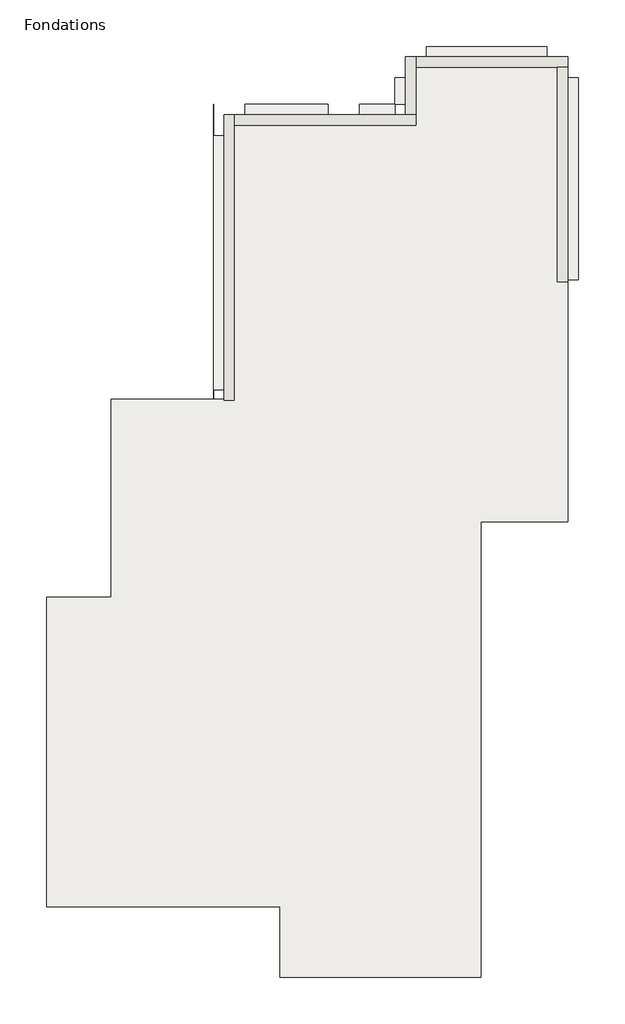
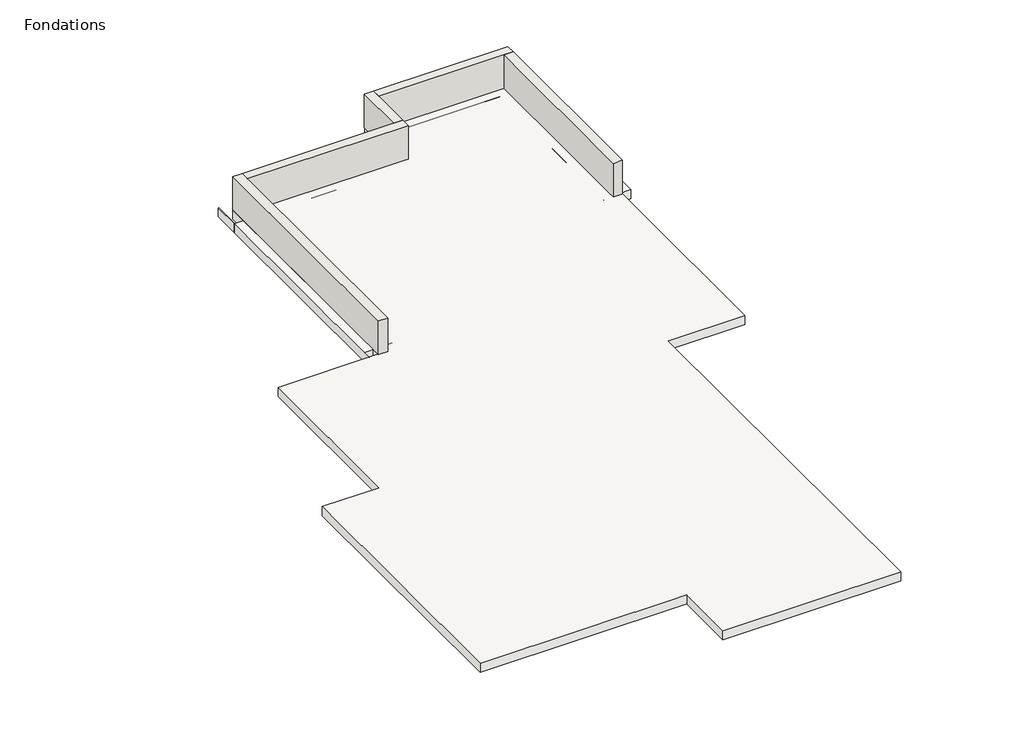
# One storey: 5 footings, 5 walls, 1 slab.
"""IFC4 building model written with IfcOpenShell, lengths in millimetres."""

from ifc_helpers import new_model, si_unit, frame, origin, place, context, project, spatial, polyline, outline, extrude, faceted_brep, element, save

model = new_model("IFC4")

# Units and contexts
model_context = context("Model", 3, world=origin())
ifc_project = project(units=[si_unit("LENGTHUNIT", "METRE", prefix="MILLI")], contexts=[model_context])

# Site, building, storey
site = spatial("IfcSite", under=ifc_project)
building = spatial("IfcBuilding", under=site)
storey = spatial("IfcBuildingStorey", under=building, Name="Fondations", Elevation=-770.0)

# Footings
placement = place(None, origin())
element("IfcFooting", 1, ObjectType="SF1 60x20ht", at=placement, inside=storey, context=model_context, shape_type="SweptSolid", body=[
    extrude(outline(polyline([(3340.0228667, 5213.5020686), (3340.0228667, 9113.5020686), (3940.0228667, 9113.5020686), (3940.0228667, 5255.0521049), (3344.5663998, 5255.0521049), (3344.5663998, 5213.5020686), (3340.0228667, 5213.5020686)])), frame((0.0, 0.0, -970.0), z_axis=(0.0, 0.0, 1.0), x_axis=(1.0, 0.0, 0.0)), (0.0, 0.0, 1.0), 200.0),
])
element("IfcFooting", 2, ObjectType="SF1 60x20ht", at=placement, inside=storey, context=model_context, shape_type="SweptSolid", body=[
    extrude(outline(polyline([(1030.0228631, 9113.5020686), (1030.0228631, 9713.5020686), (3340.0228667, 9713.5020686), (3340.0228667, 9113.5020686), (1030.0228631, 9113.5020686)])), frame((0.0, 0.0, -970.0), z_axis=(0.0, 0.0, 1.0), x_axis=(1.0, 0.0, 0.0)), (0.0, 0.0, 1.0), 200.0),
])
element("IfcFooting", 3, ObjectType="SF1 60x20ht", at=placement, inside=storey, context=model_context, shape_type="SweptSolid", body=[
    extrude(outline(polyline([(1030.0228631, 8608.0224784), (430.0228631, 8608.0224784), (430.0228631, 9113.5020686), (1030.0228631, 9113.5020686), (1030.0228631, 8608.0224784)])), frame((0.0, 0.0, -970.0), z_axis=(0.0, 0.0, 1.0), x_axis=(1.0, 0.0, 0.0)), (0.0, 0.0, 1.0), 200.0),
])
element("IfcFooting", 4, ObjectType="SF1 60x20ht", at=placement, inside=storey, context=model_context, shape_type="SweptSolid", body=[
    extrude(outline(polyline([(-2445.4336004, 8008.0224784), (-2445.4336004, 8608.0224784), (-855.4335965, 8608.0224784), (-855.4335965, 8008.0224784), (-2445.4336004, 8008.0224784)])), frame((0.0, 0.0, -970.0), z_axis=(0.0, 0.0, 1.0), x_axis=(1.0, 0.0, 0.0)), (0.0, 0.0, 1.0), 200.0),
    extrude(outline(polyline([(-255.4335965, 8008.0224784), (-255.4335965, 8608.0224784), (430.0228631, 8608.0224784), (430.0228631, 8008.0224784), (-255.4335965, 8008.0224784)])), frame((0.0, 0.0, -970.0), z_axis=(0.0, 0.0, 1.0), x_axis=(1.0, 0.0, 0.0)), (0.0, 0.0, 1.0), 200.0),
    extrude(outline(polyline([(-3049.9542111, 8008.0224784), (-3049.9542111, 8608.0224784), (-3045.4336004, 8608.0224784), (-3045.4336004, 8008.0224784), (-3049.9542111, 8008.0224784)])), frame((0.0, 0.0, -970.0), z_axis=(0.0, 0.0, 1.0), x_axis=(1.0, 0.0, 0.0)), (0.0, 0.0, 1.0), 200.0),
])
element("IfcFooting", 5, ObjectType="SF1 60x20ht", at=placement, inside=storey, context=model_context, shape_type="Brep", body=[
    faceted_brep([(-3049.9542111, 2947.3616236, -770.0), (-3049.9542111, 2947.3616236, -970.0), (-3045.4336004, 2947.3616236, -970.0), (-3045.4336004, 2947.3616236, -770.0), (-2449.9542111, 8008.0224784, -770.0), (-3045.4336004, 8008.0224784, -770.0), (-3049.9542111, 8008.0224784, -770.0), (-3045.4336004, 3148.0224782, -770.0), (-2449.9542111, 3148.0224782, -770.0), (-3049.9542111, 8008.0224784, -970.0), (-3045.4336004, 8008.0224784, -970.0), (-2449.9542111, 8008.0224784, -970.0), (-2449.9542111, 3148.0224782, -970.0), (-3045.4336004, 3148.0224782, -970.0)], [[[0, 1, 2, 3]], [[4, 5, 6, 0, 3, 7, 8]], [[1, 0, 6, 9]], [[9, 10, 11, 12, 13, 2, 1]], [[11, 4, 8, 12]], [[4, 11, 10, 9, 6, 5]], [[7, 13, 12, 8]], [[13, 7, 3, 2]]]),
])

# Slab
element("IfcSlab", 6, ObjectType="Dalla BA 20+ Fini 1", at=placement, inside=storey, context=model_context, shape_type="SweptSolid", body=[
    extrude(outline(polyline([(-2849.9542111, 2963.8353669), (-2849.9542111, 8408.0224784), (644.5663998, 8408.0224784), (644.5663998, 9513.5020686), (3740.0228667, 9513.5020686), (3740.0228667, 8408.0224784), (3740.0228667, 623.8353756), (2074.5663809, 623.8353756), (2074.5663809, -8101.9775186), (-1769.9771399, -8101.9775186), (-1769.9771399, -6748.702077), (-6246.4904445, -6748.702077), (-6246.4904445, -828.5605284), (-5012.6214092, -828.5605284), (-5012.6214092, 2963.8353669), (-2849.9542111, 2963.8353669)])), frame((0.0, 0.0, -980.0), z_axis=(0.0, 0.0, 1.0), x_axis=(1.0, 0.0, 0.0)), (0.0, 0.0, 1.0), 210.0),
])

# Walls
element("IfcWall", 7, ObjectType="Parpaing 20cm", at=placement, inside=storey, context=model_context, shape_type="Brep", body=[
    faceted_brep([(-2649.9542111, 2947.3616236, -770.0), (-2649.9542111, 8208.0224784, -770.0), (-2649.9542111, 8408.0224784, -770.0), (-2649.9542111, 8408.0224784, 0.0), (-2649.9542111, 8208.0224784, 0.0), (-2649.9542111, 2947.3616236, 0.0), (-2649.9542111, 2947.3616236, -67.0), (-2649.9542111, 2947.3616236, -767.0), (-2849.9542111, 2947.3616236, -770.0), (-2849.9542111, 2947.3616236, -767.0), (-2849.9542111, 2947.3616236, -67.0), (-2849.9542111, 2947.3616236, 0.0), (-2849.9542111, 8408.0224784, 0.0), (-2849.9542111, 8408.0224784, -770.0)], [[[0, 1, 2, 3, 4, 5, 6, 7]], [[8, 9, 10, 11, 12, 13]], [[2, 1, 0, 8, 13]], [[5, 4, 3, 12, 11]], [[0, 7, 6, 5, 11, 10, 9, 8]], [[3, 2, 13, 12]]]),
])
element("IfcWall", 8, ObjectType="Parpaing 20cm", at=placement, inside=storey, context=model_context, shape_type="Brep", body=[
    faceted_brep([(-2649.9542111, 8208.0224784, -770.0), (830.0228631, 8208.0224784, -770.0), (830.0228631, 8208.0224784, 0.0), (-2649.9542111, 8208.0224784, 0.0), (-2649.9542111, 8408.0224784, -770.0), (-2649.9542111, 8408.0224784, 0.0), (630.0228631, 8408.0224784, 0.0), (830.0228631, 8408.0224784, 0.0), (830.0228631, 8408.0224784, -770.0), (630.0228631, 8408.0224784, -770.0)], [[[0, 1, 2, 3]], [[4, 5, 6, 7, 8, 9]], [[1, 0, 4, 9, 8]], [[3, 2, 7, 6, 5]], [[2, 1, 8, 7]], [[0, 3, 5, 4]]]),
])
element("IfcWall", 9, ObjectType="Parpaing 20cm", at=placement, inside=storey, context=model_context, shape_type="Brep", body=[
    faceted_brep([(830.0228631, 8408.0224784, -770.0), (830.0228631, 9313.5020686, -770.0), (830.0228631, 9513.5020686, -770.0), (830.0228631, 9513.5020686, 0.0), (830.0228631, 9313.5020686, 0.0), (830.0228631, 8408.0224784, 0.0), (630.0228631, 8408.0224784, -770.0), (630.0228631, 8408.0224784, 0.0), (630.0228631, 9513.5020686, 0.0), (630.0228631, 9513.5020686, -770.0)], [[[0, 1, 2, 3, 4, 5]], [[6, 7, 8, 9]], [[2, 1, 0, 6, 9]], [[5, 4, 3, 8, 7]], [[0, 5, 7, 6]], [[3, 2, 9, 8]]]),
])
element("IfcWall", 10, ObjectType="Parpaing 20cm", at=placement, inside=storey, context=model_context, shape_type="Brep", body=[
    faceted_brep([(830.0228631, 9313.5020686, -770.0), (3540.0228667, 9313.5020686, -770.0), (3740.0228667, 9313.5020686, -770.0), (3740.0228667, 9313.5020686, 0.0), (3540.0228667, 9313.5020686, 0.0), (830.0228631, 9313.5020686, 0.0), (830.0228631, 9513.5020686, -770.0), (830.0228631, 9513.5020686, 0.0), (3740.0228667, 9513.5020686, 0.0), (3740.0228667, 9513.5020686, -770.0)], [[[0, 1, 2, 3, 4, 5]], [[6, 7, 8, 9]], [[2, 1, 0, 6, 9]], [[5, 4, 3, 8, 7]], [[0, 5, 7, 6]], [[3, 2, 9, 8]]]),
])
element("IfcWall", 11, ObjectType="Parpaing 20cm", at=placement, inside=storey, context=model_context, shape_type="Brep", body=[
    faceted_brep([(3540.0228667, 9313.5020686, -770.0), (3540.0228667, 5213.5020686, -770.0), (3540.0228667, 5213.5020686, 0.0), (3540.0228667, 9313.5020686, 0.0), (3740.0228667, 9313.5020686, -770.0), (3740.0228667, 9313.5020686, 0.0), (3740.0228667, 5213.5020686, 0.0), (3740.0228667, 5213.5020686, -67.0), (3740.0228667, 5213.5020686, -767.0), (3740.0228667, 5213.5020686, -770.0)], [[[0, 1, 2, 3]], [[4, 5, 6, 7, 8, 9]], [[1, 0, 4, 9]], [[2, 1, 9, 8, 7, 6]], [[3, 2, 6, 5]], [[0, 3, 5, 4]]]),
])

save(model, "model.ifc")

# Revit data of these elements
# Project information
#   Date de fin du projet = "Date de fin"
#   Etat du projet = "Etat du projet"
#   Nom du client = "Propriétaire"
#   Adresse du projet = "Entrer l'adresse ici"
#   Nom du projet = "Nom du projet"
#   Numéro de projet = "0001"
# Grids (mm)
#   "1": line (-8211.28, 9429.315) -> (5928.902, 9429.315)
#   "2": line (-8211.28, 8323.835) -> (5928.902, 8323.835)
#   "3": line (-8211.28, 7332.979) -> (5928.902, 7332.979)
#   "4": line (-8211.28, 2863.835) -> (5928.902, 2863.835)
#   "5": line (-8211.28, 523.835) -> (5928.902, 523.835)
#   "6": line (-8211.28, -928.561) -> (5928.902, -928.561)
#   "7": line (-8211.28, -2746.165) -> (5928.902, -2746.165)
#   "8": line (-8211.28, -6648.702) -> (5928.902, -6648.702)
#   "9": line (-8211.28, -7986.165) -> (5928.902, -7986.165)
#   "B": line (-4912.621, -10653.81) -> (-4912.621, 11697.731)
#   "C": line (-2745.434, -10653.81) -> (-2745.434, 12764.736)
#   "D": line (-1666.49, -10653.81) -> (-1666.49, 12114.736)
#   "E": line (-555.434, -10653.81) -> (-555.434, 12114.736)
#   "F": line (734.566, -10653.81) -> (734.566, 12114.736)
#   "G": line (1974.566, -10653.81) -> (1974.566, 12114.736)
#   "H": line (3644.566, -10653.81) -> (3644.566, 12764.736)
#   "A": line (-6146.49, -10653.81) -> (-6146.49, 11697.731)
# Type "Dalla BA 20+ Fini 1"
#   Function = 0
#   Layers, outside or top first: 0.010 m "Complexe plancher fini" (function 4); 0.200 m "Béton - Coulé sur place - Béton25" (function 1)
# Type "Parpaing 20cm"
#   Layers, outside or top first: 0.200 m "Brique, commune" (function 1)
# Elements 1, 2, 3, 4, 5 (IfcFooting, "SF1 60x20ht")
#   Phase Created = Nouvelle construction
# Element 6 (IfcSlab, "Dalla BA 20+ Fini 1")
#   Height Offset From Level = 0.000 m
#   built-in parameter 1001954 = 1
#   Phase Created = Nouvelle construction
#   Materials on its faces: "Béton - Coulé sur place - Béton25", "Complexe plancher fini"
# Elements 7, 8, 9, 10, 11 (IfcWall, "Parpaing 20cm")
#   Top Offset = 0.000 m
#   Base Offset = 0.000 m
#   wall height = 0.770 m
#   Phase Created = Nouvelle construction
#   Base Constraint = Fondations
#   Top Constraint = RDC
#   Materials on its faces: "Brique, commune"
# Materials
#   "Complexe plancher fini": class "Générique", colour RGB 120 120 120, transparency 0, Cost = 0
#   "Béton - Coulé sur place - Béton25": class "Béton", colour RGB 192 192 192, transparency 0, Cost = 0
#   "Brique, commune": class "Maçonnerie", colour RGB 85 47 55, transparency 0, Description = "Brique commune", Cost = 0
